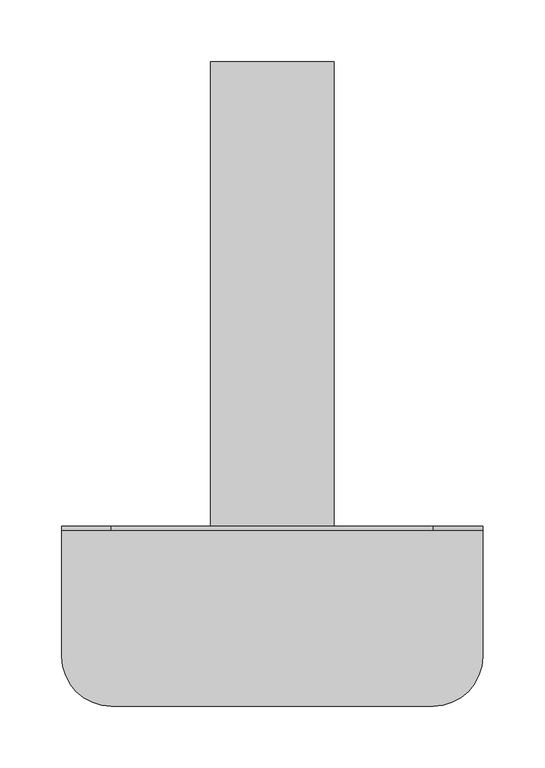
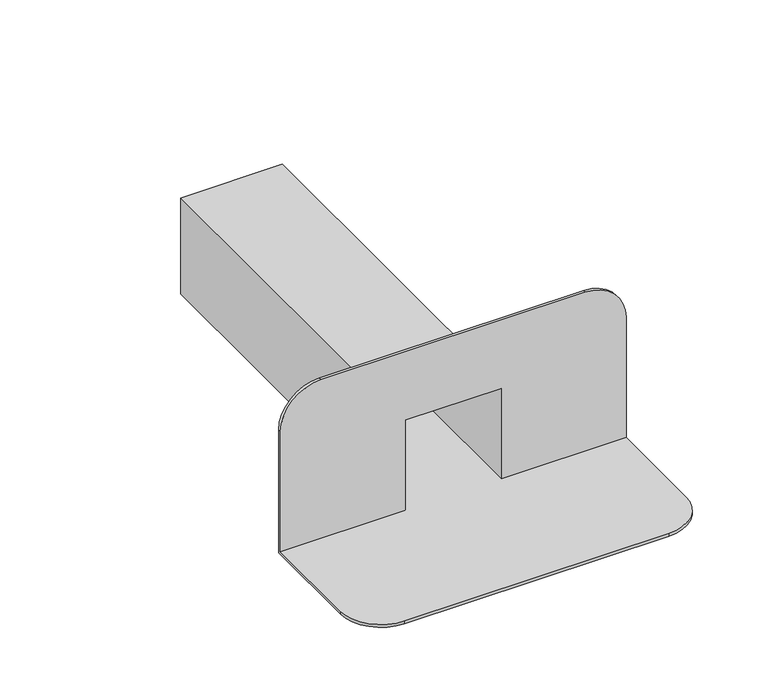
"""IFC4 building model written with IfcOpenShell, lengths in millimetres: proxy geometry, TN_Воронка парапетная ТехноНИКОЛЬ квадратная_Тип 1 : Воронка парапетная 100х100 ТехноНИКОЛЬ (квадратное сечение)."""

from ifc_helpers import new_model, si_unit, frame, origin, place, context, project, spatial, circle_curve, source, transform, mapped, element, save
from ifc_brep_helpers import plane_surface, cylinder_surface, advanced_brep


def specialty_equipment_cc57c2a0(model_context):
    return source(origin(), model_context, "Body", "AdvancedBrep", [
        advanced_brep(
        [(50.0, 375.0, 0.0), (-50.0, 375.0, 0.0), (-50.0, 375.0, 100.0), (50.0, 375.0, 100.0), (47.0, 375.0, 3.0), (47.0, 375.0, 97.0), (-47.0, 375.0, 97.0), (-47.0, 375.0, 3.0), (50.0, 0.0, 100.0), (50.0, 0.0, 0.0), (-50.0, 0.0, 100.0), (-50.0, 0.0, 0.0), (170.0, 0.0, 0.0), (170.0, -105.0, 0.0), (130.0, -145.0, 0.0), (-130.0, -145.0, 0.0), (-170.0, -105.0, 0.0), (-170.0, 0.0, 0.0), (-47.0, -3.0, 3.0), (-170.0, -3.0, 3.0), (-170.0, -105.0, 3.0), (-130.0, -145.0, 3.0), (130.0, -145.0, 3.0), (170.0, -105.0, 3.0), (170.0, -3.0, 3.0), (47.0, -3.0, 3.0), (-47.0, -3.0, 97.0), (47.0, -3.0, 97.0), (170.0, -3.0, 128.0), (130.0, -3.0, 168.0), (-130.0, -3.0, 168.0), (-170.0, -3.0, 128.0), (-170.0, 0.0, 128.0), (-130.0, 0.0, 168.0), (130.0, 0.0, 168.0), (170.0, 0.0, 128.0)],
        [
            (0, 1),
            (1, 2),
            (2, 3),
            (3, 0),
            (4, 5),
            (5, 6),
            (6, 7),
            (7, 4),
            (3, 8),
            (8, 9),
            (9, 0),
            (2, 10),
            (10, 8),
            (1, 11),
            (11, 10),
            (9, 12),
            (12, 13),
            (13, 14, circle_curve(frame((130.0, -105.0, 0.0), z_axis=(0.0, 0.0, -1.0), x_axis=(1.0, 0.0, 0.0)), 40.0)),
            (14, 15),
            (15, 16, circle_curve(frame((-130.0, -105.0, 0.0), z_axis=(0.0, 0.0, -1.0), x_axis=(1.0, 0.0, 0.0)), 40.0)),
            (16, 17),
            (17, 11),
            (7, 18),
            (18, 19),
            (19, 20),
            (20, 21, circle_curve(frame((-130.0, -105.0, 3.0), z_axis=(0.0, 0.0, 1.0), x_axis=(1.0, 0.0, 0.0)), 40.0)),
            (21, 22),
            (22, 23, circle_curve(frame((130.0, -105.0, 3.0), z_axis=(0.0, 0.0, 1.0), x_axis=(1.0, 0.0, 0.0)), 40.0)),
            (23, 24),
            (24, 25),
            (25, 4),
            (6, 26),
            (26, 18),
            (5, 27),
            (27, 26),
            (25, 27),
            (24, 28),
            (28, 29, circle_curve(frame((130.0, -3.0, 128.0), z_axis=(0.0, -1.0, 0.0), x_axis=(1.0, 0.0, 0.0)), 40.0)),
            (29, 30),
            (30, 31, circle_curve(frame((-130.0, -3.0, 128.0), z_axis=(0.0, -1.0, 0.0), x_axis=(1.0, 0.0, 0.0)), 40.0)),
            (31, 19),
            (32, 33, circle_curve(frame((-130.0, 0.0, 128.0), z_axis=(0.0, 1.0, 0.0), x_axis=(1.0, 0.0, 0.0)), 40.0)),
            (33, 34),
            (34, 35, circle_curve(frame((130.0, 0.0, 128.0), z_axis=(0.0, 1.0, 0.0), x_axis=(1.0, 0.0, 0.0)), 40.0)),
            (35, 12),
            (17, 32),
            (23, 13),
            (35, 28),
            (34, 29),
            (33, 30),
            (32, 31),
            (16, 20),
            (15, 21),
            (14, 22),
        ],
        [
            plane_surface(frame((50.0, 375.0, 0.0), z_axis=(0.0, 1.0, 0.0), x_axis=(0.0, 0.0, -1.0))),
            plane_surface(frame((50.0, 0.0, 0.0), z_axis=(1.0, 0.0, 0.0), x_axis=(0.0, 1.0, 0.0))),
            plane_surface(frame((50.0, 0.0, 100.0), z_axis=(0.0, 0.0, 1.0), x_axis=(0.0, 1.0, 0.0))),
            plane_surface(frame((-50.0, 0.0, 100.0), z_axis=(-1.0, 0.0, 0.0), x_axis=(0.0, 1.0, 0.0))),
            plane_surface(frame((-50.0, 0.0, 0.0), z_axis=(0.0, 0.0, -1.0), x_axis=(0.0, 1.0, 0.0))),
            plane_surface(frame((47.0, 0.0, 3.0), z_axis=(0.0, 0.0, 1.0), x_axis=(0.0, 1.0, 0.0))),
            plane_surface(frame((-47.0, 0.0, 3.0), z_axis=(1.0, 0.0, 0.0), x_axis=(0.0, 1.0, 0.0))),
            plane_surface(frame((-47.0, 0.0, 97.0), z_axis=(0.0, 0.0, -1.0), x_axis=(0.0, 1.0, 0.0))),
            plane_surface(frame((47.0, 0.0, 97.0), z_axis=(-1.0, 0.0, 0.0), x_axis=(0.0, 1.0, 0.0))),
            plane_surface(frame((170.0, -3.0, 128.0), z_axis=(0.0, -1.0, 0.0), x_axis=(0.0, 0.0, 1.0))),
            plane_surface(frame((170.0, 0.0, 128.0), z_axis=(0.0, 1.0, 0.0), x_axis=(0.0, 0.0, -1.0))),
            plane_surface(frame((170.0, -3.0, 3.0), z_axis=(1.0, 0.0, 0.0), x_axis=(0.0, 1.0, 0.0))),
            cylinder_surface(frame((130.0, 0.0, 128.0), z_axis=(0.0, -1.0, 0.0), x_axis=(1.0, 0.0, 0.0)), 40.0),
            plane_surface(frame((130.0, -3.0, 168.0), z_axis=(0.0, 0.0, 1.0), x_axis=(0.0, 1.0, 0.0))),
            cylinder_surface(frame((-130.0, 0.0, 128.0), z_axis=(0.0, -1.0, 0.0), x_axis=(1.0, 0.0, 0.0)), 40.0),
            plane_surface(frame((-170.0, -3.0, 128.0), z_axis=(-1.0, 0.0, 0.0), x_axis=(0.0, 1.0, 0.0))),
            cylinder_surface(frame((-130.0, -105.0, 0.0), z_axis=(0.0, 0.0, 1.0), x_axis=(1.0, 0.0, 0.0)), 40.0),
            plane_surface(frame((-130.0, -145.0, 3.0), z_axis=(0.0, -1.0, 0.0), x_axis=(0.0, 0.0, -1.0))),
            cylinder_surface(frame((130.0, -105.0, 0.0), z_axis=(0.0, 0.0, 1.0), x_axis=(1.0, 0.0, 0.0)), 40.0),
        ],
        [
            (0, [[1, 2, 3, 4], [5, 6, 7, 8]]),
            (1, [[-4, 9, 10, 11]]),
            (2, [[-3, 12, 13, -9]]),
            (3, [[-2, 14, 15, -12]]),
            (4, [[-1, -11, 16, 17, 18, 19, 20, 21, 22, -14]]),
            (5, [[-8, 23, 24, 25, 26, 27, 28, 29, 30, 31]]),
            (6, [[-23, -7, 32, 33]]),
            (7, [[-6, 34, 35, -32]]),
            (8, [[-5, -31, 36, -34]]),
            (9, [[37, 38, 39, 40, 41, -24, -33, -35, -36, -30]]),
            (10, [[42, 43, 44, 45, -16, -10, -13, -15, -22, 46]]),
            (11, [[-37, -29, 47, -17, -45, 48]]),
            (12, [[-38, -48, -44, 49]]),
            (13, [[-39, -49, -43, 50]]),
            (14, [[-40, -50, -42, 51]]),
            (15, [[-41, -51, -46, -21, 52, -25]]),
            (16, [[-26, -52, -20, 53]]),
            (17, [[-27, -53, -19, 54]]),
            (18, [[-28, -54, -18, -47]]),
        ],
    ),
    ])


if __name__ == "__main__":
    model = new_model("IFC4")
    model_context = context("Model", 3, world=origin())
    ifc_project = project(units=[si_unit("LENGTHUNIT", "METRE", prefix="MILLI")], contexts=[model_context])
    site = spatial("IfcSite", under=ifc_project)
    building = spatial("IfcBuilding", under=site)
    placement = place(None, origin())
    specialty_equipment_shape = specialty_equipment_cc57c2a0(model_context)
    element("IfcBuildingElementProxy", 1, Name="TN_Воронка парапетная ТехноНИКОЛЬ квадратная_Тип 1 : Воронка парапетная 100х100 ТехноНИКОЛЬ (квадратное сечение)", ObjectType="TN_Воронка парапетная ТехноНИКОЛЬ квадратная_Тип 1 : Воронка парапетная 100х100 ТехноНИКОЛЬ (квадратное сечение)", at=placement, inside=building, context=model_context, shape_type="MappedRepresentation", body=[
        mapped(specialty_equipment_shape, transform((0.0, 0.0, 0.0), x_axis=(1.0, 0.0, 0.0), y_axis=(0.0, 1.0, 0.0), z_axis=(0.0, 0.0, 1.0))),
    ])
    save(model, "model.ifc")

# Revit data of these elements
# Type "TN_Воронка парапетная ТехноНИКОЛЬ квадратная_Тип 1 : Воронка парапетная 100х100 ТехноНИКОЛЬ (квадратное сечение)"
#   ADSK_Группирование = "Комплектующие и воронки"
#   Description = "Воронка парапетная 100х100 – воронка для организации внешнего водостока через балконы и парапеты на пониженных участках кровли. Воронка имеет квадратное сечение отводящей трубы. Используются при строительстве и реконструкции зданий и сооружений. Применяется в плоских кровлях из битумных и битумно-полимерных рулонных материалов с внешним водостоком через балконы и парапеты кровли. Пропуская способность 8 л/сек."
#   Manufacturer = "ТехноНИКОЛЬ"
#   URL = "http://nav.tn.ru/catalog/krovlya/vodostochnaya-sistema/parapetnaya-voronka-tekhnonikol/"
#   ADSK_Примечание = ""
#   ADSK_Обозначение = "ТехноНИКОЛЬ"
#   ADSK_Наименование = "Воронка парапетная 100х100 ТехноНИКОЛЬ (квадратное сечение)"
#   ADSK_Марка = ""
#   ADSK_Код изделия = "467191"
#   ADSK_Завод-изготовитель = "ТехноНИКОЛЬ"
#   ADSK_Единица измерения = "шт."
#   ADSK_Группирование = "Комплектующие и воронки"
#   ADSK_URL страницы изделия = ""
#   ADSK_URL документации изделия = ""
#   Ширина фланца = 340 mm
#   Размер фланца по вертикали = 168 mm
#   Длина расчетная [instance default] = 375 mm
#   Длина отвода [instance default] = 375 mm
#   Размер фланца по горизонтали = 145 mm
#   ADSK_Масса = 1.25
#   ADSK_Количество = 1
#   Видимость_Переход [instance default] = yes
#   Материал = TN_ПВХ_Черный
#   Default Elevation = 0
# Element 1 (IfcBuildingElementProxy, "TN_Воронка парапетная ТехноНИКОЛЬ квадратная_Тип 1 : Воронка парапетная 100х100 ТехноНИКОЛЬ (квадратное сечение)")
#   Видимость_Переход = no
#   Materials on its faces: "TN_ПВХ_Черный"
# Materials
#   "TN_ПВХ_Черный": class "Типовые", colour RGB 48 48 48, transparency 0, Cost = 0
